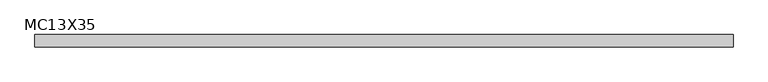
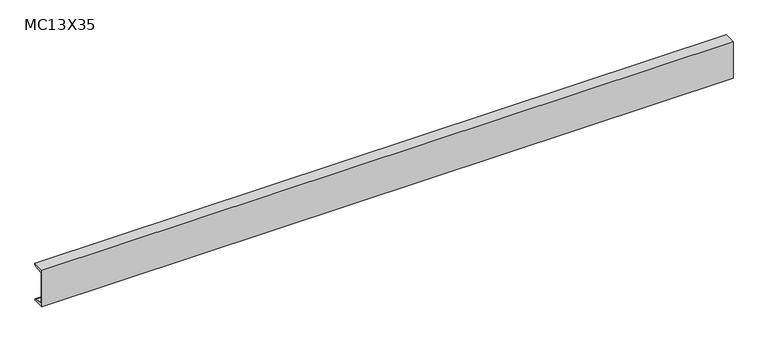
"""IFC4 building model written with IfcOpenShell, lengths in millimetres: beam geometry, MC-Miscellaneous Channel : MC13X35."""

from ifc_helpers import new_model, si_unit, point, frame, frame_2d, origin, place, context, project, spatial, polyline, circle_curve, trimmed, segment, composite_curve, outline, extrude, source, transform, mapped, element, save


def mc13x35_48cd5bcc(model_context):
    return source(origin(), model_context, "Body", "SweptSolid", [
        extrude(outline(composite_curve([segment(polyline([(-24.892, 165.1), (78.486, 165.1)]), True, "CONTINUOUS"), segment(trimmed(circle_curve(frame_2d((62.992, 165.1)), 15.494), [point((78.486, 165.1))], [point((62.992, 149.606))], False, "CARTESIAN"), True, "CONTINUOUS"), segment(polyline([(62.992, 149.606), (-13.5382, 137.4848071), (-13.5382, -137.4848071), (62.992, -149.606)]), True, "CONTINUOUS"), segment(trimmed(circle_curve(frame_2d((62.992, -165.1)), 15.494), [point((62.992, -149.606))], [point((78.486, -165.1))], False, "CARTESIAN"), True, "CONTINUOUS"), segment(polyline([(78.486, -165.1), (-24.892, -165.1), (-24.892, 165.1)]), True, "CONTINUOUS")], self_intersect=False)), frame((-3082.798, 0.0, 0.0), z_axis=(1.0, 0.0, 0.0), x_axis=(0.0, 1.0, 0.0)), (0.0, 0.0, 1.0), 5914.898),
    ])


if __name__ == "__main__":
    model = new_model("IFC4")
    model_context = context("Model", 3, world=origin())
    ifc_project = project(units=[si_unit("LENGTHUNIT", "METRE", prefix="MILLI")], contexts=[model_context])
    site = spatial("IfcSite", under=ifc_project)
    building = spatial("IfcBuilding", under=site)
    placement = place(None, origin())
    mc13x35_shape = mc13x35_48cd5bcc(model_context)
    element("IfcBeam", 1, ObjectType="MC-Miscellaneous Channel : MC13X35", at=placement, inside=building, context=model_context, shape_type="MappedRepresentation", body=[
        mapped(mc13x35_shape, transform((0.0, 0.0, 0.0), x_axis=(1.0, 0.0, 0.0), y_axis=(0.0, 1.0, 0.0), z_axis=(0.0, 0.0, 1.0))),
    ])
    save(model, "model.ifc")

# Revit data of these elements
# Type "MC-Miscellaneous Channel : MC13X35"
#   Assembly Code = "B10"
#   W = 35
#   Length [instance default] = 5' - 0"
#   bf = 0' - 4.07"
#   d = 1' - 1"
#   tf = 0' - 0.61"
#   tw = 0' - 0.447"
#   x = 0' - 0.98"
#   A = 0.0715278 SF
#   Structural Material [instance default] = Steel ASTM A36
# Element 1 (IfcBeam, "MC-Miscellaneous Channel : MC13X35")
#   Structural Material = Steel ASTM A992
#   Materials on its faces: "Steel ASTM A992"
# Materials
#   "Steel ASTM A36": class "Metal", colour RGB 199 199 199, transparency 0, Description = "Structural steel, ASTM A36 Grade B, mill finish", Cost = 0
#   "Steel ASTM A992": class "Metal", colour RGB 199 199 199, transparency 0, Description = "Structural steel 50ksi", Cost = 0
